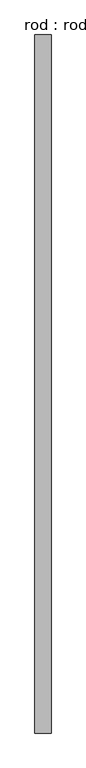
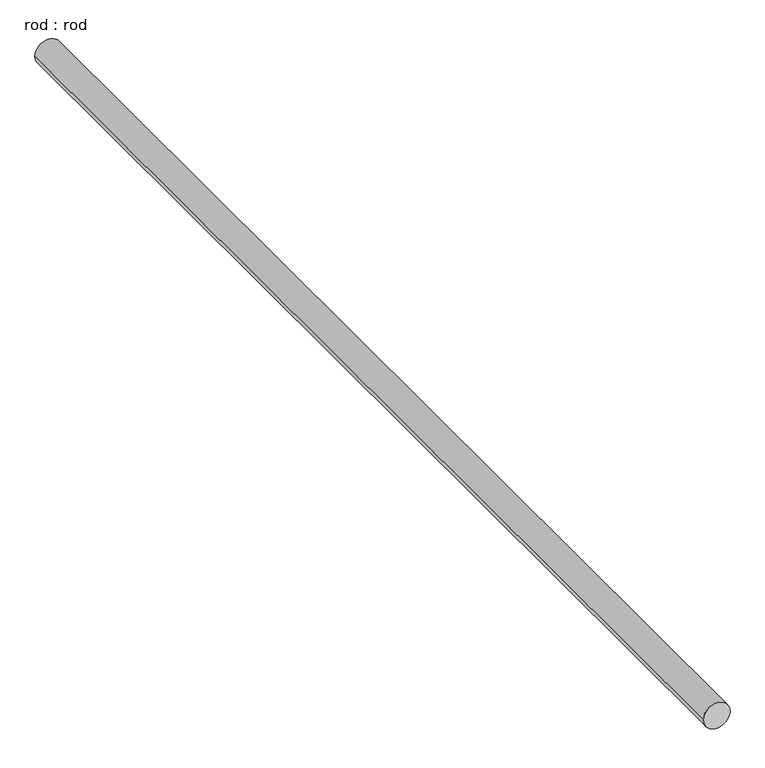
"""IFC4 building model written with IfcOpenShell, lengths in millimetres: proxy geometry, rod : rod."""

from ifc_helpers import new_model, si_unit, point, frame, frame_2d, origin, place, context, project, spatial, circle_curve, trimmed, segment, composite_curve, outline, extrude, source, transform, mapped, element, save


def rod_rod_69e40952(model_context):
    return source(origin(), model_context, "Body", "SweptSolid", [
        extrude(outline(composite_curve([segment(trimmed(circle_curve(frame_2d((0.0108462, 0.0)), 200.0), [point((0.0108462, 200.0))], [point((0.0108462, -200.0))], False, "CARTESIAN"), True, "CONTINUOUS"), segment(trimmed(circle_curve(frame_2d((0.0108462, 0.0)), 200.0), [point((0.0108462, -200.0))], [point((0.0108462, 200.0))], False, "CARTESIAN"), True, "CONTINUOUS")], self_intersect=False)), frame((0.0, -4549.208469, 0.0), z_axis=(0.0, 1.0, 0.0), x_axis=(0.0, 0.0, 1.0)), (0.0, 0.0, 1.0), 17283.8741688),
    ])


if __name__ == "__main__":
    model = new_model("IFC4")
    model_context = context("Model", 3, world=origin())
    ifc_project = project(units=[si_unit("LENGTHUNIT", "METRE", prefix="MILLI")], contexts=[model_context])
    site = spatial("IfcSite", under=ifc_project)
    building = spatial("IfcBuilding", under=site)
    placement = place(None, origin())
    rod_rod_shape = rod_rod_69e40952(model_context)
    element("IfcBuildingElementProxy", 1, Name="rod : rod", ObjectType="rod : rod", at=placement, inside=building, context=model_context, shape_type="MappedRepresentation", body=[
        mapped(rod_rod_shape, transform((0.0, 0.0, 0.0), x_axis=(1.0, 0.0, 0.0), y_axis=(0.0, 1.0, 0.0), z_axis=(0.0, 0.0, 1.0))),
    ])
    save(model, "model.ifc")

# Revit data of these elements
# Type "rod : rod"
#   Default Elevation = 0
